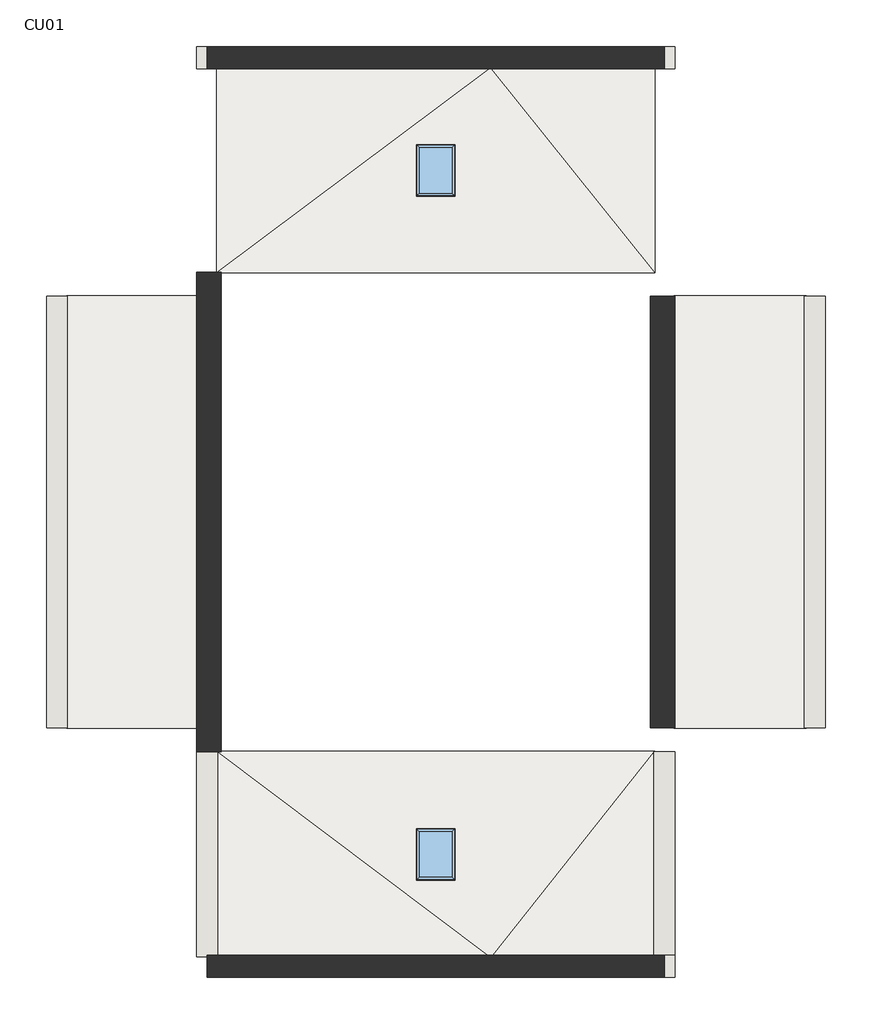
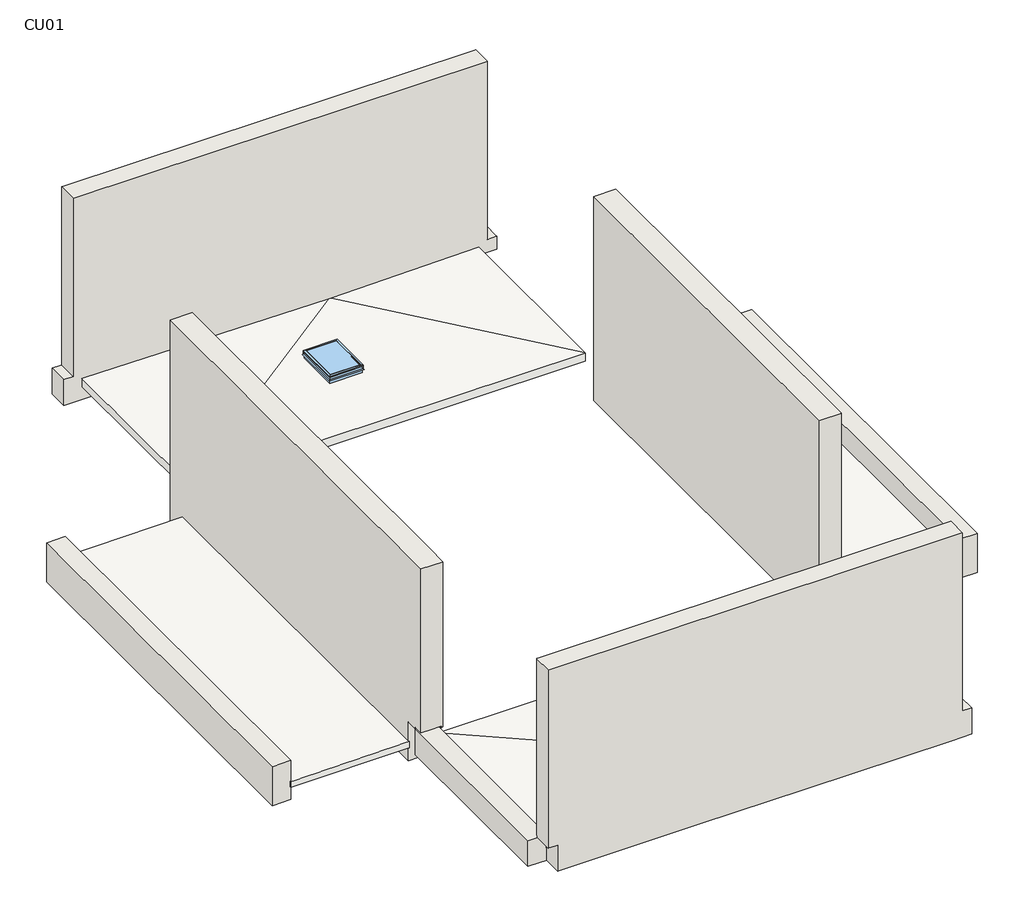
# One storey: 8 walls, 4 roofs, 2 windows.
# Revit data of these elements (continued)
# Materials (continued)
#   "Lana de vidrio": class "Genérico", colour RGB 120 120 120, transparency 0, Comments = "Aislamiento térmico (6 cm)", Description = "Lana de fibra de vidrio", Cost = 0
#   "Cámara de aire": class "Gas", colour RGB 183 255 255, transparency 0.75, Description = "Aire", Cost = 0
#   "Enlucido de yeso": class "Placa de yeso laminado", colour RGB 249 249 249, transparency 0, Keynote = "1", Comments = "Color blanco al temple (1,5 cm)", Description = "1", Cost = 0
#   "Metal - Bronce, Bruñido ligero": class "Metal", colour RGB 113 80 70, transparency 0
#   "Vidrio": class "Vidrio", colour RGB 0 128 192, transparency 0.75, Description = "Vidrio de cal sodada", Cost = 0
#   "Muro por defecto": class "Varios", colour RGB 212 212 212, transparency 0, Cost = 0
